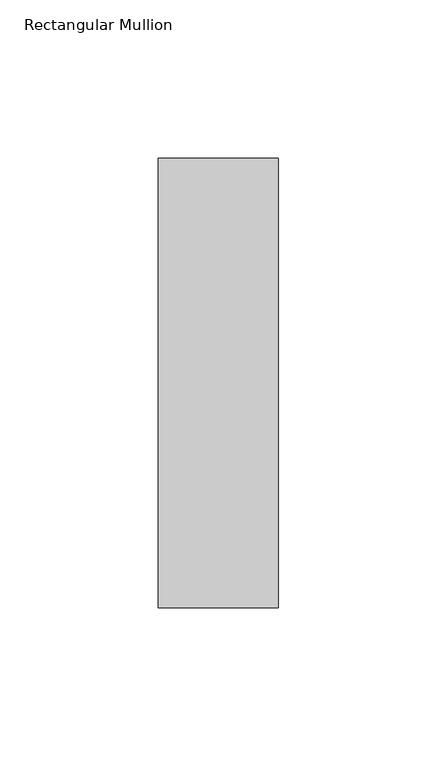
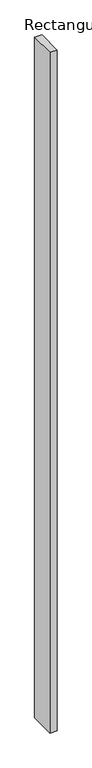
"""IFC4 building model written with IfcOpenShell, lengths in millimetres: member geometry, Rectangular Mullion : NLRS_21_CWM_hsb-regel 38x142_gen_rsf."""

import ifcopenshell
import ifcopenshell.guid

model = None  # the IFC model being written
_history = None  # IfcOwnerHistory: only IFC2X3 demands one
_inside = {}  # id of a spatial element -> (the spatial element, [elements in it])
_under = {}  # id of a project, library or spatial element -> (it, [spatial elements below it])
_declared = {}  # id of a project -> (the project, [libraries it declares])
_typed = {}  # id of a type object -> (the type object, [elements of that type])
_made_of = {}  # id of a material, layer set ... -> (it, [elements and type objects made of it])


def new_model(schema):
    """Start an empty IFC model of exactly this schema.

    Asked for "IFC4X3", IfcOpenShell would pick the latest addendum, in which some entities
    have other attributes; the version numbers below select the first issue.
    IFC2X3 requires an IfcOwnerHistory on every rooted entity: one is made here for all.
    """
    global model, _history
    if schema == "IFC4X3":
        model = ifcopenshell.file(schema_version=(4, 3, 0, 0))
    else:
        model = ifcopenshell.file(schema=schema)
    _inside.clear()
    _under.clear()
    _declared.clear()
    _typed.clear()
    _made_of.clear()
    _history = None
    if model.schema == "IFC2X3":
        org = make("IfcOrganization", Name="unknown")
        user = make(
            "IfcPersonAndOrganization",
            ThePerson=make("IfcPerson", FamilyName="unknown"),
            TheOrganization=org,
        )
        app = make(
            "IfcApplication",
            ApplicationDeveloper=org,
            Version="unknown",
            ApplicationFullName="unknown",
            ApplicationIdentifier="unknown",
        )
        _history = make(
            "IfcOwnerHistory",
            OwningUser=user,
            OwningApplication=app,
            ChangeAction="ADDED",
            CreationDate=0,
        )
    return model


def make(cls, **values):
    """One entity of the class cls with the attributes given. An attribute that is None is left unset."""
    return model.create_entity(
        cls, **{name: value for name, value in values.items() if value is not None}
    )


def rooted(cls, **values):
    """An entity with a GlobalId (a new one), such as an element, a storey or a relation."""
    return make(cls, GlobalId=ifcopenshell.guid.new(), OwnerHistory=_history, **values)


def si_unit(unit_type, name, prefix=None):
    """IfcSIUnit, for example si_unit("LENGTHUNIT", "METRE", prefix="MILLI")."""
    return make("IfcSIUnit", UnitType=unit_type, Prefix=prefix, Name=name)


def assignment(units):
    """IfcUnitAssignment: the units of a project."""
    return None if units is None else make("IfcUnitAssignment", Units=units)


def point(xyz):
    """IfcCartesianPoint."""
    return None if xyz is None else make("IfcCartesianPoint", Coordinates=xyz)


def direction(xyz):
    """IfcDirection."""
    return None if xyz is None else make("IfcDirection", DirectionRatios=xyz)


def frame(location, z_axis=None, x_axis=None):
    """IfcAxis2Placement3D, a coordinate frame: its origin and axes. An axis left out is left unset."""
    return make(
        "IfcAxis2Placement3D",
        Location=point(location),
        Axis=direction(z_axis),
        RefDirection=direction(x_axis),
    )


def origin():
    """The frame at (0, 0, 0) with its axes left unset."""
    return frame((0.0, 0.0, 0.0))


def place(relative_to, where):
    """IfcLocalPlacement: puts the frame where relative to a parent placement (None: the world)."""
    return make(
        "IfcLocalPlacement", PlacementRelTo=relative_to, RelativePlacement=where
    )


def context(
    kind, dimensions, precision=None, world=None, true_north=None, identifier=None
):
    """IfcGeometricRepresentationContext, for example the 3D "Model" context."""
    return make(
        "IfcGeometricRepresentationContext",
        ContextIdentifier=identifier,
        ContextType=kind,
        CoordinateSpaceDimension=dimensions,
        Precision=precision,
        WorldCoordinateSystem=world,
        TrueNorth=true_north,
    )


def project(units=None, contexts=None):
    """IfcProject with its units and contexts."""
    return rooted(
        "IfcProject",
        Name="project",
        RepresentationContexts=contexts,
        UnitsInContext=assignment(units),
    )


def spatial(cls, under=None, at=None, **own):
    """A site, building, storey or space (cls), placed at a placement, below another one or the project."""
    s = rooted(cls, ObjectPlacement=at, **own)
    if under is not None:
        _under.setdefault(under.id(), (under, []))[1].append(s)
    return s


def polyline(points):
    """IfcPolyline through the points."""
    return make("IfcPolyline", Points=[point(p) for p in points])


def outline(outer, holes=None, kind="AREA"):
    """IfcArbitraryClosedProfileDef: a profile drawn as a closed curve; with holes, ...WithVoids."""
    if holes is None:
        return make("IfcArbitraryClosedProfileDef", ProfileType=kind, OuterCurve=outer)
    return make(
        "IfcArbitraryProfileDefWithVoids",
        ProfileType=kind,
        OuterCurve=outer,
        InnerCurves=holes,
    )


def extrude(swept, where, along, depth):
    """IfcExtrudedAreaSolid: the profile swept, set in the frame where, extruded along a direction by depth."""
    return make(
        "IfcExtrudedAreaSolid",
        SweptArea=swept,
        Position=where,
        ExtrudedDirection=direction(along),
        Depth=depth,
    )


def shape(context_of_items, identifier, shape_type, items):
    """IfcShapeRepresentation: the items that make up one representation, for example the "Body"."""
    return make(
        "IfcShapeRepresentation",
        ContextOfItems=context_of_items,
        RepresentationIdentifier=identifier,
        RepresentationType=shape_type,
        Items=items,
    )


def source(mapping_origin, context_of_items, identifier, shape_type, items):
    """IfcRepresentationMap: a shape defined once, which mapped items show again and again."""
    return make(
        "IfcRepresentationMap",
        MappingOrigin=mapping_origin,
        MappedRepresentation=shape(context_of_items, identifier, shape_type, items),
    )


def transform(
    local_origin,
    x_axis=None,
    y_axis=None,
    z_axis=None,
    scale=None,
    scale2=None,
    scale3=None,
    uniform=True,
):
    """IfcCartesianTransformationOperator3D, or its non-uniform kind. x_axis, y_axis, z_axis: its Axis1, 2, 3."""
    if uniform:
        return make(
            "IfcCartesianTransformationOperator3D",
            Axis1=direction(x_axis),
            Axis2=direction(y_axis),
            LocalOrigin=point(local_origin),
            Scale=scale,
            Axis3=direction(z_axis),
        )
    return make(
        "IfcCartesianTransformationOperator3DnonUniform",
        Axis1=direction(x_axis),
        Axis2=direction(y_axis),
        LocalOrigin=point(local_origin),
        Scale=scale,
        Axis3=direction(z_axis),
        Scale2=scale2,
        Scale3=scale3,
    )


def mapped(mapping_source, mapping_target):
    """IfcMappedItem: shows the shape of a source again, moved by a transform."""
    return make(
        "IfcMappedItem", MappingSource=mapping_source, MappingTarget=mapping_target
    )


def made_of(thing, what):
    """Note that an element or type object is made of a material, layer set ...; save() writes the relation."""
    if what is not None:
        _made_of.setdefault(what.id(), (what, []))[1].append(thing)
    return thing


def element(
    cls,
    number,
    at=None,
    inside=None,
    cuts=None,
    type_object=None,
    material=None,
    context=None,
    identifier="Body",
    shape_type=None,
    held_by="IfcProductDefinitionShape",
    body=None,
    shapes=None,
    **own,
):
    """One element of the class cls, such as IfcWall. Its Tag is "e" and its number.

    at: its placement. inside: the storey or other place that contains it. cuts: it is an
    opening in that element (IfcRelVoidsElement). A single representation is given by context,
    identifier, shape_type and body (its items); several are given by shapes. held_by: the class
    of the entity that holds the representations. save() writes the other relations.
    """
    e = rooted(cls, Tag="e%d" % number, ObjectPlacement=at, **own)
    if body is not None:
        shapes = [shape(context, identifier, shape_type, body)]
    if shapes is not None:
        e.Representation = make(held_by, Representations=shapes)
    if inside is not None:
        _inside.setdefault(inside.id(), (inside, []))[1].append(e)
    if cuts is not None:
        rooted(
            "IfcRelVoidsElement", RelatingBuildingElement=cuts, RelatedOpeningElement=e
        )
    if type_object is not None:
        _typed.setdefault(type_object.id(), (type_object, []))[1].append(e)
    return made_of(e, material)


def aggregate(whole, parts):
    """IfcRelAggregates: a whole, such as a stair, and the parts it consists of."""
    return rooted("IfcRelAggregates", RelatingObject=whole, RelatedObjects=parts)


def save(model, path):
    """Write the relations noted so far, then the file.

    IfcRelAggregates (storeys below a building ...), IfcRelContainedInSpatialStructure (elements
    in a storey), IfcRelDefinesByType, IfcRelAssociatesMaterial and IfcRelDeclares: one each for
    every whole, place, type object, material and project.
    """
    for whole, parts in _under.values():
        aggregate(whole, parts)
    for where, things in _inside.values():
        rooted(
            "IfcRelContainedInSpatialStructure",
            RelatedElements=things,
            RelatingStructure=where,
        )
    for kind, things in _typed.values():
        rooted("IfcRelDefinesByType", RelatedObjects=things, RelatingType=kind)
    for what, things in _made_of.values():
        rooted("IfcRelAssociatesMaterial", RelatedObjects=things, RelatingMaterial=what)
    for by, libraries in _declared.values():
        rooted("IfcRelDeclares", RelatingContext=by, RelatedDefinitions=libraries)
    model.write(path)


def rectangular_mullion_bc699282(model_context):
    return source(origin(), model_context, "Body", "SweptSolid", [
        extrude(outline(polyline([(19.0, -71.0), (-19.0, -71.0), (-19.0, 71.0), (19.0, 71.0), (19.0, -71.0)])), frame((0.0, 0.0, -3849.0), z_axis=(0.0, 0.0, 1.0), x_axis=(1.0, 0.0, 0.0)), (0.0, 0.0, 1.0), 3849.0),
    ])


if __name__ == "__main__":
    model = new_model("IFC4")
    model_context = context("Model", 3, world=origin())
    ifc_project = project(units=[si_unit("LENGTHUNIT", "METRE", prefix="MILLI")], contexts=[model_context])
    site = spatial("IfcSite", under=ifc_project)
    building = spatial("IfcBuilding", under=site)
    placement = place(None, origin())
    rectangular_mullion_shape = rectangular_mullion_bc699282(model_context)
    element("IfcMember", 1, ObjectType="Rectangular Mullion : NLRS_21_CWM_hsb-regel 38x142_gen_rsf", at=placement, inside=building, context=model_context, shape_type="MappedRepresentation", body=[
        mapped(rectangular_mullion_shape, transform((0.0, 0.0, 0.0), x_axis=(1.0, 0.0, 0.0), y_axis=(0.0, 1.0, 0.0), z_axis=(0.0, 0.0, 1.0))),
    ])
    save(model, "model.ifc")

# Revit data of these elements
# Type "Rectangular Mullion : NLRS_21_CWM_hsb-regel 38x142_gen_rsf"
#   Export Type to IFC As = "IfcWall"
#   Type IfcGUID = "07M7mRoiH1CR8m_RSKIwpF"
#   Assembly Code = "21.10"
#   built-in parameter 1007322 = 0.465879 (stored number, unit not read)
#   built-in parameter 1007321 = 0.062336 (stored number, unit not read)
#   built-in parameter 1007320 = 0.062336 (stored number, unit not read)
# Element 1 (IfcMember, "Rectangular Mullion : NLRS_21_CWM_hsb-regel 38x142_gen_rsf")
#   Materials on its faces: "NLRS_i2_hout naaldhout vuren_gen_rsf"
# Materials
#   "NLRS_i2_hout naaldhout vuren_gen_rsf": class "I - Hout", colour RGB 234 199 147, transparency 0, Keynote = "i2", Manufacturer = "Revit Standards Foundation", URL = "www.revitstandards.org", Description = "hout vuren", Cost = 0
